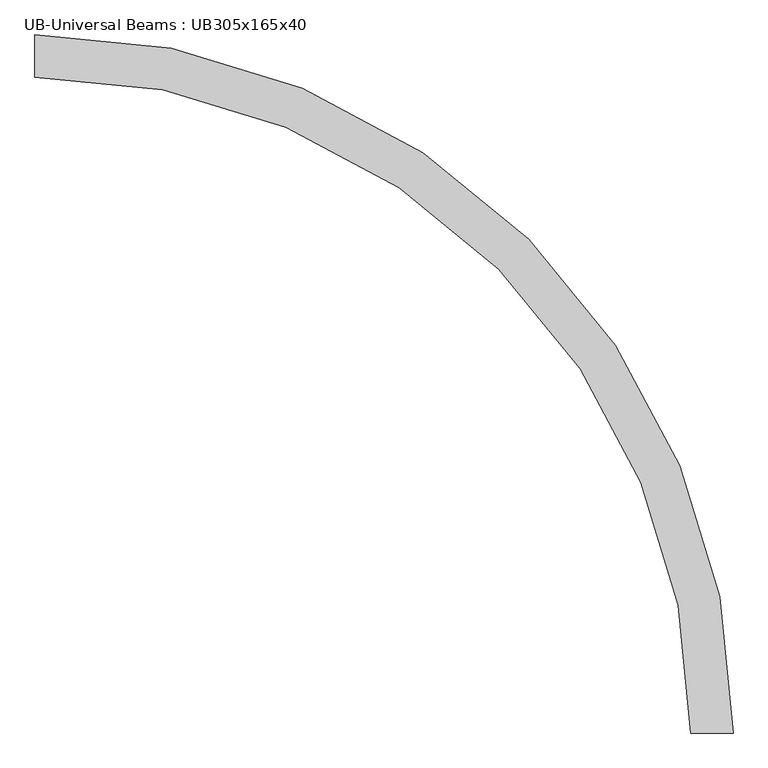
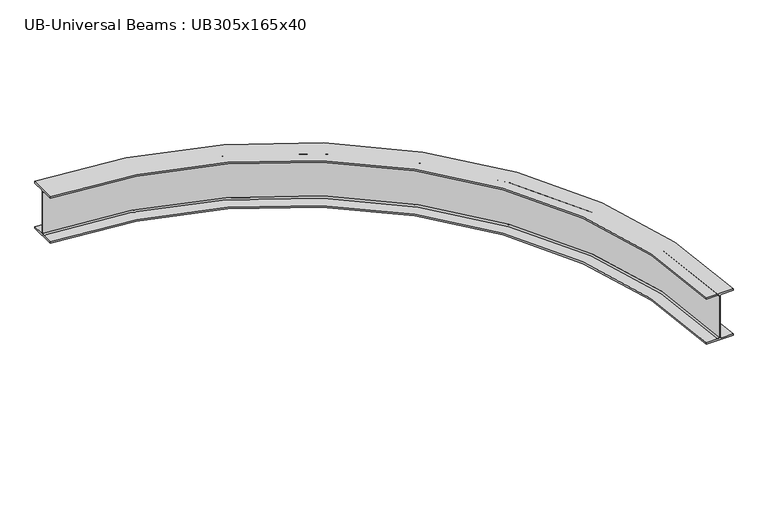
"""IFC4 building model written with IfcOpenShell, lengths in millimetres: beam geometry, UB-Universal Beams : UB305x165x40."""

import ifcopenshell
import ifcopenshell.guid

model = None  # the IFC model being written
_history = None  # IfcOwnerHistory: only IFC2X3 demands one
_inside = {}  # id of a spatial element -> (the spatial element, [elements in it])
_under = {}  # id of a project, library or spatial element -> (it, [spatial elements below it])
_declared = {}  # id of a project -> (the project, [libraries it declares])
_typed = {}  # id of a type object -> (the type object, [elements of that type])
_made_of = {}  # id of a material, layer set ... -> (it, [elements and type objects made of it])


def new_model(schema):
    """Start an empty IFC model of exactly this schema.

    Asked for "IFC4X3", IfcOpenShell would pick the latest addendum, in which some entities
    have other attributes; the version numbers below select the first issue.
    IFC2X3 requires an IfcOwnerHistory on every rooted entity: one is made here for all.
    """
    global model, _history
    if schema == "IFC4X3":
        model = ifcopenshell.file(schema_version=(4, 3, 0, 0))
    else:
        model = ifcopenshell.file(schema=schema)
    _inside.clear()
    _under.clear()
    _declared.clear()
    _typed.clear()
    _made_of.clear()
    _history = None
    if model.schema == "IFC2X3":
        org = make("IfcOrganization", Name="unknown")
        user = make(
            "IfcPersonAndOrganization",
            ThePerson=make("IfcPerson", FamilyName="unknown"),
            TheOrganization=org,
        )
        app = make(
            "IfcApplication",
            ApplicationDeveloper=org,
            Version="unknown",
            ApplicationFullName="unknown",
            ApplicationIdentifier="unknown",
        )
        _history = make(
            "IfcOwnerHistory",
            OwningUser=user,
            OwningApplication=app,
            ChangeAction="ADDED",
            CreationDate=0,
        )
    return model


def make(cls, **values):
    """One entity of the class cls with the attributes given. An attribute that is None is left unset."""
    return model.create_entity(
        cls, **{name: value for name, value in values.items() if value is not None}
    )


def rooted(cls, **values):
    """An entity with a GlobalId (a new one), such as an element, a storey or a relation."""
    return make(cls, GlobalId=ifcopenshell.guid.new(), OwnerHistory=_history, **values)


def si_unit(unit_type, name, prefix=None):
    """IfcSIUnit, for example si_unit("LENGTHUNIT", "METRE", prefix="MILLI")."""
    return make("IfcSIUnit", UnitType=unit_type, Prefix=prefix, Name=name)


def assignment(units):
    """IfcUnitAssignment: the units of a project."""
    return None if units is None else make("IfcUnitAssignment", Units=units)


def point(xyz):
    """IfcCartesianPoint."""
    return None if xyz is None else make("IfcCartesianPoint", Coordinates=xyz)


def direction(xyz):
    """IfcDirection."""
    return None if xyz is None else make("IfcDirection", DirectionRatios=xyz)


def frame(location, z_axis=None, x_axis=None):
    """IfcAxis2Placement3D, a coordinate frame: its origin and axes. An axis left out is left unset."""
    return make(
        "IfcAxis2Placement3D",
        Location=point(location),
        Axis=direction(z_axis),
        RefDirection=direction(x_axis),
    )


def origin():
    """The frame at (0, 0, 0) with its axes left unset."""
    return frame((0.0, 0.0, 0.0))


def place(relative_to, where):
    """IfcLocalPlacement: puts the frame where relative to a parent placement (None: the world)."""
    return make(
        "IfcLocalPlacement", PlacementRelTo=relative_to, RelativePlacement=where
    )


def context(
    kind, dimensions, precision=None, world=None, true_north=None, identifier=None
):
    """IfcGeometricRepresentationContext, for example the 3D "Model" context."""
    return make(
        "IfcGeometricRepresentationContext",
        ContextIdentifier=identifier,
        ContextType=kind,
        CoordinateSpaceDimension=dimensions,
        Precision=precision,
        WorldCoordinateSystem=world,
        TrueNorth=true_north,
    )


def project(units=None, contexts=None):
    """IfcProject with its units and contexts."""
    return rooted(
        "IfcProject",
        Name="project",
        RepresentationContexts=contexts,
        UnitsInContext=assignment(units),
    )


def spatial(cls, under=None, at=None, **own):
    """A site, building, storey or space (cls), placed at a placement, below another one or the project."""
    s = rooted(cls, ObjectPlacement=at, **own)
    if under is not None:
        _under.setdefault(under.id(), (under, []))[1].append(s)
    return s


def polyline(points):
    """IfcPolyline through the points."""
    return make("IfcPolyline", Points=[point(p) for p in points])


def circle_curve(where, radius):
    """IfcCircle in the frame where."""
    return make("IfcCircle", Position=where, Radius=radius)


def ellipse_curve(where, semi_axis1, semi_axis2):
    """IfcEllipse in the frame where."""
    return make(
        "IfcEllipse", Position=where, SemiAxis1=semi_axis1, SemiAxis2=semi_axis2
    )


def trimmed(basis, trim1, trim2, sense, master):
    """IfcTrimmedCurve: the piece of a basis curve between two trims."""
    return make(
        "IfcTrimmedCurve",
        BasisCurve=basis,
        Trim1=trim1,
        Trim2=trim2,
        SenseAgreement=sense,
        MasterRepresentation=master,
    )


def shape(context_of_items, identifier, shape_type, items):
    """IfcShapeRepresentation: the items that make up one representation, for example the "Body"."""
    return make(
        "IfcShapeRepresentation",
        ContextOfItems=context_of_items,
        RepresentationIdentifier=identifier,
        RepresentationType=shape_type,
        Items=items,
    )


def source(mapping_origin, context_of_items, identifier, shape_type, items):
    """IfcRepresentationMap: a shape defined once, which mapped items show again and again."""
    return make(
        "IfcRepresentationMap",
        MappingOrigin=mapping_origin,
        MappedRepresentation=shape(context_of_items, identifier, shape_type, items),
    )


def transform(
    local_origin,
    x_axis=None,
    y_axis=None,
    z_axis=None,
    scale=None,
    scale2=None,
    scale3=None,
    uniform=True,
):
    """IfcCartesianTransformationOperator3D, or its non-uniform kind. x_axis, y_axis, z_axis: its Axis1, 2, 3."""
    if uniform:
        return make(
            "IfcCartesianTransformationOperator3D",
            Axis1=direction(x_axis),
            Axis2=direction(y_axis),
            LocalOrigin=point(local_origin),
            Scale=scale,
            Axis3=direction(z_axis),
        )
    return make(
        "IfcCartesianTransformationOperator3DnonUniform",
        Axis1=direction(x_axis),
        Axis2=direction(y_axis),
        LocalOrigin=point(local_origin),
        Scale=scale,
        Axis3=direction(z_axis),
        Scale2=scale2,
        Scale3=scale3,
    )


def mapped(mapping_source, mapping_target):
    """IfcMappedItem: shows the shape of a source again, moved by a transform."""
    return make(
        "IfcMappedItem", MappingSource=mapping_source, MappingTarget=mapping_target
    )


def made_of(thing, what):
    """Note that an element or type object is made of a material, layer set ...; save() writes the relation."""
    if what is not None:
        _made_of.setdefault(what.id(), (what, []))[1].append(thing)
    return thing


def element(
    cls,
    number,
    at=None,
    inside=None,
    cuts=None,
    type_object=None,
    material=None,
    context=None,
    identifier="Body",
    shape_type=None,
    held_by="IfcProductDefinitionShape",
    body=None,
    shapes=None,
    **own,
):
    """One element of the class cls, such as IfcWall. Its Tag is "e" and its number.

    at: its placement. inside: the storey or other place that contains it. cuts: it is an
    opening in that element (IfcRelVoidsElement). A single representation is given by context,
    identifier, shape_type and body (its items); several are given by shapes. held_by: the class
    of the entity that holds the representations. save() writes the other relations.
    """
    e = rooted(cls, Tag="e%d" % number, ObjectPlacement=at, **own)
    if body is not None:
        shapes = [shape(context, identifier, shape_type, body)]
    if shapes is not None:
        e.Representation = make(held_by, Representations=shapes)
    if inside is not None:
        _inside.setdefault(inside.id(), (inside, []))[1].append(e)
    if cuts is not None:
        rooted(
            "IfcRelVoidsElement", RelatingBuildingElement=cuts, RelatedOpeningElement=e
        )
    if type_object is not None:
        _typed.setdefault(type_object.id(), (type_object, []))[1].append(e)
    return made_of(e, material)


def aggregate(whole, parts):
    """IfcRelAggregates: a whole, such as a stair, and the parts it consists of."""
    return rooted("IfcRelAggregates", RelatingObject=whole, RelatedObjects=parts)


def save(model, path):
    """Write the relations noted so far, then the file.

    IfcRelAggregates (storeys below a building ...), IfcRelContainedInSpatialStructure (elements
    in a storey), IfcRelDefinesByType, IfcRelAssociatesMaterial and IfcRelDeclares: one each for
    every whole, place, type object, material and project.
    """
    for whole, parts in _under.values():
        aggregate(whole, parts)
    for where, things in _inside.values():
        rooted(
            "IfcRelContainedInSpatialStructure",
            RelatedElements=things,
            RelatingStructure=where,
        )
    for kind, things in _typed.values():
        rooted("IfcRelDefinesByType", RelatedObjects=things, RelatingType=kind)
    for what, things in _made_of.values():
        rooted("IfcRelAssociatesMaterial", RelatedObjects=things, RelatingMaterial=what)
    for by, libraries in _declared.values():
        rooted("IfcRelDeclares", RelatingContext=by, RelatedDefinitions=libraries)
    model.write(path)


def plane_surface(at):
    """IfcPlane: the flat surface through the origin of the frame at, square to its z axis."""
    return make("IfcPlane", Position=at)


def cylinder_surface(at, radius):
    """IfcCylindricalSurface: all points at the distance radius from the z axis of the frame at."""
    return make("IfcCylindricalSurface", Position=at, Radius=radius)


def revolved_surface(curve, axis_point, axis_direction):
    """IfcSurfaceOfRevolution: the curve turned about the line through axis_point along axis_direction."""
    return make(
        "IfcSurfaceOfRevolution",
        SweptCurve=make("IfcArbitraryOpenProfileDef", ProfileType="CURVE", Curve=curve),
        AxisPosition=make("IfcAxis1Placement", Location=point(axis_point), Axis=direction(axis_direction)),
    )


def advanced_brep(points, edges, surfaces, faces):
    """IfcAdvancedBrep: a solid bounded by faces that lie on surfaces and meet in shared edges.

    An edge is (start, end): straight between two places in points (the first is 0);
    or (start, end, curve); or (start, end, curve, False) where it runs against its curve.
    A face is (place in surfaces, loops), or (place, loops, False) where it looks against
    its surface's normal. A loop lists edges by number (the first is 1), with a minus sign
    where the edge is run from its end to its start. The first loop is the outer one.
    """
    corners = [point(p) for p in points]
    vertices = [make("IfcVertexPoint", VertexGeometry=c) for c in corners]
    made = []
    for start, end, *more in edges:
        made.append(
            make(
                "IfcEdgeCurve",
                EdgeStart=vertices[start],
                EdgeEnd=vertices[end],
                EdgeGeometry=more[0] if more else make("IfcPolyline", Points=[corners[start], corners[end]]),
                SameSense=more[1] if len(more) > 1 else True,
            )
        )
    hull = []
    for where, loops, *sense in faces:
        bounds = []
        for j, loop in enumerate(loops):
            ring = [make("IfcOrientedEdge", EdgeElement=made[abs(k) - 1], Orientation=k > 0) for k in loop]
            bounds.append(
                make(
                    "IfcFaceOuterBound" if j == 0 else "IfcFaceBound",
                    Bound=make("IfcEdgeLoop", EdgeList=ring),
                    Orientation=True,
                )
            )
        hull.append(make("IfcAdvancedFace", Bounds=bounds, FaceSurface=surfaces[where], SameSense=sense[0] if sense else True))
    return make("IfcAdvancedBrep", Outer=make("IfcClosedShell", CfsFaces=hull))


def ub_universal_beams_ub305x165x40_a7bc032b(model_context):
    return source(origin(), model_context, "Body", "AdvancedBrep", [
        advanced_brep(
        [(2724.4689627, -2641.9689627, -141.5), (2653.8689627, -2641.9689627, -141.5), (2644.9689627, -2641.9689627, -132.6), (2644.9689627, -2641.9689627, 132.6), (2653.8689627, -2641.9689627, 141.5), (2724.4689627, -2641.9689627, 141.5), (2724.4689627, -2641.9689627, 151.7), (2559.4689627, -2641.9689627, 151.7), (2559.4689627, -2641.9689627, 141.5), (2630.0689627, -2641.9689627, 141.5), (2638.9689627, -2641.9689627, 132.6), (2638.9689627, -2641.9689627, -132.6), (2630.0689627, -2641.9689627, -141.5), (2559.4689627, -2641.9689627, -141.5), (2559.4689627, -2641.9689627, -151.7), (2724.4689627, -2641.9689627, -151.7), (0.0, 82.5, -141.5), (0.0, 82.5, -151.7), (0.0, -82.5, -151.7), (0.0, -82.5, -141.5), (0.0, -11.9, -141.5), (0.0, -3.0, -132.6), (0.0, -3.0, 132.6), (0.0, -11.9, 141.5), (0.0, -82.5, 141.5), (0.0, -82.5, 151.7), (0.0, 82.5, 151.7), (0.0, 82.5, 141.5), (0.0, 11.9, 141.5), (0.0, 3.0, 132.6), (0.0, 3.0, -132.6), (0.0, 11.9, -141.5)],
        [
            (0, 1),
            (1, 2, circle_curve(frame((2653.8689627, -2641.9689627, -132.6), z_axis=(0.0, 1.0, 0.0), x_axis=(-1.0, 0.0, 0.0)), 8.9)),
            (2, 3),
            (3, 4, circle_curve(frame((2653.8689627, -2641.9689627, 132.6), z_axis=(0.0, 1.0, 0.0), x_axis=(-1.0, 0.0, 0.0)), 8.9)),
            (4, 5),
            (5, 6),
            (6, 7),
            (7, 8),
            (8, 9),
            (9, 10, circle_curve(frame((2630.0689627, -2641.9689627, 132.6), z_axis=(0.0, 1.0, 0.0), x_axis=(-1.0, 0.0, 0.0)), 8.9)),
            (10, 11),
            (11, 12, circle_curve(frame((2630.0689627, -2641.9689627, -132.6), z_axis=(0.0, 1.0, 0.0), x_axis=(-1.0, 0.0, 0.0)), 8.9)),
            (12, 13),
            (13, 14),
            (14, 15),
            (15, 0),
            (16, 17),
            (17, 18),
            (18, 19),
            (19, 20),
            (20, 21, circle_curve(frame((0.0, -11.9, -132.6), z_axis=(1.0, 0.0, 0.0), x_axis=(0.0, -1.0, 0.0)), 8.9)),
            (21, 22),
            (22, 23, circle_curve(frame((0.0, -11.9, 132.6), z_axis=(1.0, 0.0, 0.0), x_axis=(0.0, -1.0, 0.0)), 8.9)),
            (23, 24),
            (24, 25),
            (25, 26),
            (26, 27),
            (27, 28),
            (28, 29, circle_curve(frame((0.0, 11.9, 132.6), z_axis=(1.0, 0.0, 0.0), x_axis=(0.0, -1.0, 0.0)), 8.9)),
            (29, 30),
            (30, 31, circle_curve(frame((0.0, 11.9, -132.6), z_axis=(1.0, 0.0, 0.0), x_axis=(0.0, -1.0, 0.0)), 8.9)),
            (31, 16),
            (0, 16, circle_curve(frame((0.0, -2641.9689627, -141.5), z_axis=(0.0, 0.0, 1.0), x_axis=(0.0, 1.0, 0.0)), 2724.4689627)),
            (31, 1, circle_curve(frame((0.0, -2641.9689627, -141.5), z_axis=(0.0, 0.0, -1.0), x_axis=(0.0, 1.0, 0.0)), 2653.8689627)),
            (30, 2, circle_curve(frame((0.0, -2641.9689627, -132.6), z_axis=(0.0, 0.0, -1.0), x_axis=(0.0, 1.0, 0.0)), 2644.9689627)),
            (29, 3, circle_curve(frame((0.0, -2641.9689627, 132.6), z_axis=(0.0, 0.0, -1.0), x_axis=(0.0, 1.0, 0.0)), 2644.9689627)),
            (28, 4, circle_curve(frame((0.0, -2641.9689627, 141.5), z_axis=(0.0, 0.0, -1.0), x_axis=(0.0, 1.0, 0.0)), 2653.8689627)),
            (27, 5, circle_curve(frame((0.0, -2641.9689627, 141.5), z_axis=(0.0, 0.0, -1.0), x_axis=(0.0, 1.0, 0.0)), 2724.4689627)),
            (26, 6, circle_curve(frame((0.0, -2641.9689627, 151.7), z_axis=(0.0, 0.0, -1.0), x_axis=(0.0, 1.0, 0.0)), 2724.4689627)),
            (25, 7, circle_curve(frame((0.0, -2641.9689627, 151.7), z_axis=(0.0, 0.0, -1.0), x_axis=(0.0, 1.0, 0.0)), 2559.4689627)),
            (24, 8, circle_curve(frame((0.0, -2641.9689627, 141.5), z_axis=(0.0, 0.0, -1.0), x_axis=(0.0, 1.0, 0.0)), 2559.4689627)),
            (23, 9, circle_curve(frame((0.0, -2641.9689627, 141.5), z_axis=(0.0, 0.0, -1.0), x_axis=(0.0, 1.0, 0.0)), 2630.0689627)),
            (22, 10, circle_curve(frame((0.0, -2641.9689627, 132.6), z_axis=(0.0, 0.0, -1.0), x_axis=(0.0, 1.0, 0.0)), 2638.9689627)),
            (21, 11, circle_curve(frame((0.0, -2641.9689627, -132.6), z_axis=(0.0, 0.0, -1.0), x_axis=(0.0, 1.0, 0.0)), 2638.9689627)),
            (20, 12, circle_curve(frame((0.0, -2641.9689627, -141.5), z_axis=(0.0, 0.0, -1.0), x_axis=(0.0, 1.0, 0.0)), 2630.0689627)),
            (19, 13, circle_curve(frame((0.0, -2641.9689627, -141.5), z_axis=(0.0, 0.0, -1.0), x_axis=(0.0, 1.0, 0.0)), 2559.4689627)),
            (18, 14, circle_curve(frame((0.0, -2641.9689627, -151.7), z_axis=(0.0, 0.0, -1.0), x_axis=(0.0, 1.0, 0.0)), 2559.4689627)),
            (17, 15, circle_curve(frame((0.0, -2641.9689627, -151.7), z_axis=(0.0, 0.0, -1.0), x_axis=(0.0, 1.0, 0.0)), 2724.4689627)),
        ],
        [
            plane_surface(frame((2641.9689627, -2641.9689627, 0.0), z_axis=(0.0, -1.0, 0.0), x_axis=(0.0, 0.0, 1.0))),
            plane_surface(frame((0.0, 0.0, 0.0), z_axis=(-1.0, 0.0, 0.0), x_axis=(0.0, 0.0, 1.0))),
            plane_surface(frame((0.0, -2641.9689627, -141.5), z_axis=(0.0, 0.0, 1.0), x_axis=(0.0, 1.0, 0.0))),
            revolved_surface(trimmed(ellipse_curve(frame((0.0, 11.9, -132.6), z_axis=(1.0, 0.0, 0.0), x_axis=(0.0, -1.0, 0.0)), 8.9, 8.9), [point((0.0, 3.0, -132.6))], [point((0.0, 11.9, -141.5))], True, "CARTESIAN"), (0.0, -2641.9689627, 0.0), (0.0, 0.0, -1.0)),
            cylinder_surface(frame((0.0, -2641.9689627, 0.0), z_axis=(0.0, 0.0, -1.0), x_axis=(0.0, 1.0, 0.0)), 2644.9689627),
            revolved_surface(trimmed(ellipse_curve(frame((0.0, 11.9, 132.6), z_axis=(1.0, 0.0, 0.0), x_axis=(0.0, -1.0, 0.0)), 8.9, 8.9), [point((0.0, 11.9, 141.5))], [point((0.0, 3.0, 132.6))], True, "CARTESIAN"), (0.0, -2641.9689627, 0.0), (0.0, 0.0, -1.0)),
            plane_surface(frame((0.0, -2641.9689627, 141.5), z_axis=(0.0, 0.0, -1.0), x_axis=(0.0, 1.0, 0.0))),
            cylinder_surface(frame((0.0, -2641.9689627, 0.0), z_axis=(0.0, 0.0, -1.0), x_axis=(0.0, 1.0, 0.0)), 2724.4689627),
            plane_surface(frame((0.0, -2641.9689627, 151.7), z_axis=(0.0, 0.0, 1.0), x_axis=(0.0, 1.0, 0.0))),
            revolved_surface(polyline([(0.0, -82.5, 141.5), (0.0, -82.5, 151.7)]), (0.0, -2641.9689627, 0.0), (0.0, 0.0, -1.0)),
            revolved_surface(trimmed(ellipse_curve(frame((0.0, -11.9, 132.6), z_axis=(1.0, 0.0, 0.0), x_axis=(0.0, -1.0, 0.0)), 8.9, 8.9), [point((0.0, -3.0, 132.6))], [point((0.0, -11.9, 141.5))], True, "CARTESIAN"), (0.0, -2641.9689627, 0.0), (0.0, 0.0, -1.0)),
            revolved_surface(polyline([(0.0, -3.0, -132.6), (0.0, -3.0, 132.6)]), (0.0, -2641.9689627, 0.0), (0.0, 0.0, -1.0)),
            revolved_surface(trimmed(ellipse_curve(frame((0.0, -11.9, -132.6), z_axis=(1.0, 0.0, 0.0), x_axis=(0.0, -1.0, 0.0)), 8.9, 8.9), [point((0.0, -11.9, -141.5))], [point((0.0, -3.0, -132.6))], True, "CARTESIAN"), (0.0, -2641.9689627, 0.0), (0.0, 0.0, -1.0)),
            revolved_surface(polyline([(0.0, -82.5, -151.7), (0.0, -82.5, -141.5)]), (0.0, -2641.9689627, 0.0), (0.0, 0.0, -1.0)),
            plane_surface(frame((0.0, -2641.9689627, -151.7), z_axis=(0.0, 0.0, -1.0), x_axis=(0.0, 1.0, 0.0))),
        ],
        [
            (0, [[1, 2, 3, 4, 5, 6, 7, 8, 9, 10, 11, 12, 13, 14, 15, 16]]),
            (1, [[17, 18, 19, 20, 21, 22, 23, 24, 25, 26, 27, 28, 29, 30, 31, 32]]),
            (2, [[-1, 33, -32, 34]]),
            (3, [[-2, -34, -31, 35]]),
            (4, [[-3, -35, -30, 36]]),
            (5, [[-4, -36, -29, 37]]),
            (6, [[-5, -37, -28, 38]]),
            (7, [[-6, -38, -27, 39]]),
            (8, [[-7, -39, -26, 40]]),
            (9, [[-8, -40, -25, 41]]),
            (6, [[-9, -41, -24, 42]]),
            (10, [[-10, -42, -23, 43]]),
            (11, [[-11, -43, -22, 44]]),
            (12, [[-12, -44, -21, 45]]),
            (2, [[-13, -45, -20, 46]]),
            (13, [[-14, -46, -19, 47]]),
            (14, [[-15, -47, -18, 48]]),
            (7, [[-16, -48, -17, -33]]),
        ],
    ),
    ])


if __name__ == "__main__":
    model = new_model("IFC4")
    model_context = context("Model", 3, world=origin())
    ifc_project = project(units=[si_unit("LENGTHUNIT", "METRE", prefix="MILLI")], contexts=[model_context])
    site = spatial("IfcSite", under=ifc_project)
    building = spatial("IfcBuilding", under=site)
    placement = place(None, origin())
    ub_universal_beams_ub305x165x40_shape = ub_universal_beams_ub305x165x40_a7bc032b(model_context)
    element("IfcBeam", 1, ObjectType="UB-Universal Beams : UB305x165x40", at=placement, inside=building, context=model_context, shape_type="MappedRepresentation", body=[
        mapped(ub_universal_beams_ub305x165x40_shape, transform((0.0, 0.0, 0.0), x_axis=(1.0, 0.0, 0.0), y_axis=(0.0, 1.0, 0.0), z_axis=(0.0, 0.0, 1.0))),
    ])
    save(model, "model.ifc")

# Revit data of these elements
# Type "UB-Universal Beams : UB305x165x40"
#   Section Name Key = "UB305X165X40"
#   Width = 16.5 cm
#   Web Thickness = 0.6 cm
#   Web Fillet = 0.89 cm
#   Warping Constant = 164000.0 cm⁶
#   Torsional Moment of Inertia = 14.70 cm⁴
#   Section Area = 51.3 cm²
#   Plastic Modulus weak axis = 142.0 cm³
#   Plastic Modulus strong axis = 623.0 cm³
#   Nominal Weight = 40.2999 kgf/m
#   Moment of Inertia weak axis = 764.00 cm⁴
#   Moment of Inertia strong axis = 8503.00 cm⁴
#   Height = 30.34 cm
#   Flange Thickness = 1.02 cm
#   Elastic Modulus weak axis = 92.6 cm³
#   Elastic Modulus strong axis = 560.0 cm³
#   Centroid Vertical = 15.17 cm
#   Centroid Horizontal = 8.25 cm
#   Bolt Spacing = 9.0 cm
#   Length [instance default] = 1500 mm
#   Structural Material [instance default] = Metal - Steel 43-275
#   Type Comments = ""
#   Assembly Code = ""
# Element 1 (IfcBeam, "UB-Universal Beams : UB305x165x40")
#   Materials on its faces: "Metal - Steel 43-275"
# Materials
#   "Metal - Steel 43-275": class "Metal", colour RGB 247 247 247, transparency 0, Cost = 0
